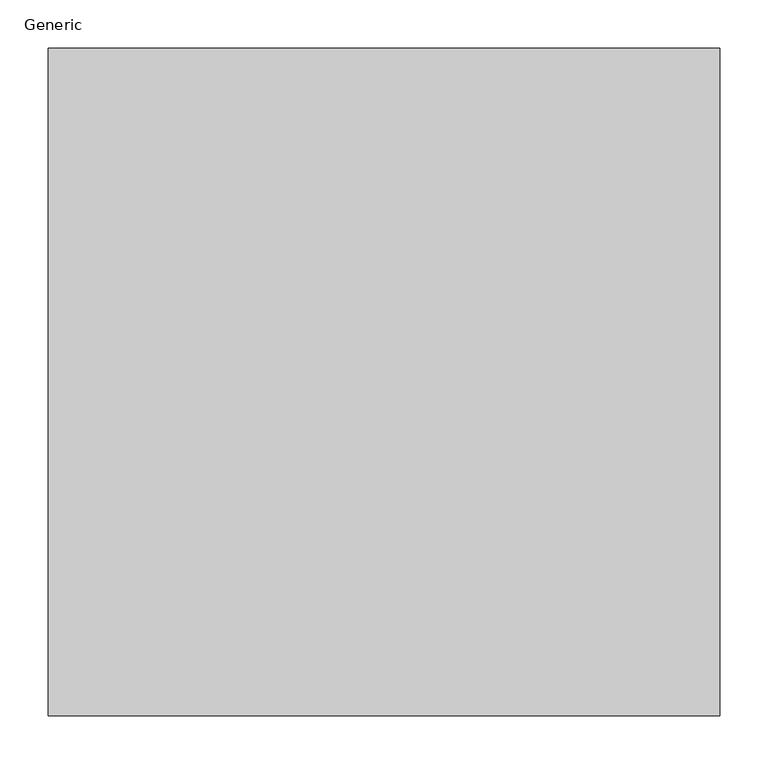
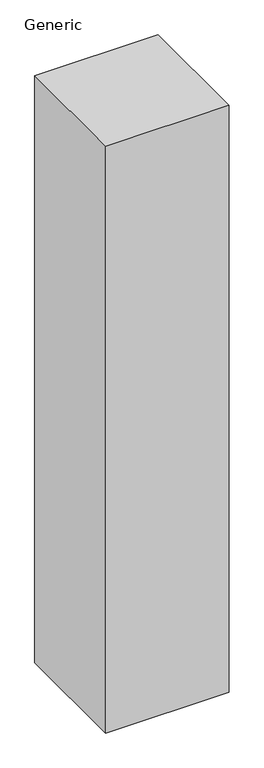
"""IFC4 building model written with IfcOpenShell, lengths in millimetres: column geometry, WWm-ConcreteRectangular-Instance : Generic."""

from ifc_helpers import new_model, si_unit, origin, origin_with_axes, place, context, project, spatial, polyline, outline, extrude, source, transform, mapped, element, save


def generic_81af98c7(model_context):
    return source(origin(), model_context, "Body", "SweptSolid", [
        extrude(outline(polyline([(391.2, 387.2), (391.2, -304.8), (-304.8, -304.8), (-304.8, 387.2), (391.2, 387.2)])), origin_with_axes(), (0.0, 0.0, 1.0), 3500.0),
    ])


if __name__ == "__main__":
    model = new_model("IFC4")
    model_context = context("Model", 3, world=origin())
    ifc_project = project(units=[si_unit("LENGTHUNIT", "METRE", prefix="MILLI")], contexts=[model_context])
    site = spatial("IfcSite", under=ifc_project)
    building = spatial("IfcBuilding", under=site)
    placement = place(None, origin())
    generic_shape = generic_81af98c7(model_context)
    element("IfcColumn", 1, ObjectType="WWm-ConcreteRectangular-Instance : Generic", at=placement, inside=building, context=model_context, shape_type="MappedRepresentation", body=[
        mapped(generic_shape, transform((0.0, 0.0, 0.0), x_axis=(1.0, 0.0, 0.0), y_axis=(0.0, 1.0, 0.0), z_axis=(0.0, 0.0, 1.0))),
    ])
    save(model, "model.ifc")

# Revit data of these elements
# Type "WWm-ConcreteRectangular-Instance : Generic"
#   Depth [instance default] = 600 mm
#   Offset Base = 0 mm
#   Offset Top = 0 mm
#   Width [instance default] = 600 mm
#   Material = WW-EC-CR-CastInPlace
#   Assembly Code = ""
# Element 1 (IfcColumn, "WWm-ConcreteRectangular-Instance : Generic")
#   Depth = 692 mm
#   Width = 696 mm
#   Materials on its faces: "WW-EC-CR-CastInPlace"
# Materials
#   "WW-EC-CR-CastInPlace": class "Concrete", colour RGB 255 255 255, transparency 0, Comments = "If region requests all-white model, remove image from asset", Description = "Cast in Place Concrete", Cost = 0
